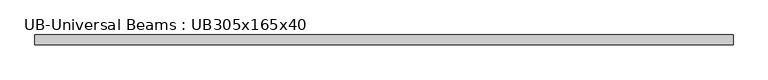
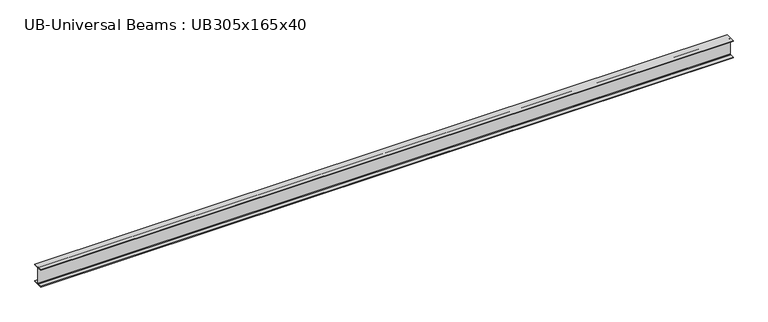
"""IFC4 building model written with IfcOpenShell, lengths in millimetres: member geometry, UB-Universal Beams : UB305x165x40."""

from ifc_helpers import new_model, si_unit, point, frame, frame_2d, origin, place, context, project, spatial, polyline, circle_curve, trimmed, segment, composite_curve, outline, extrude, source, transform, mapped, element, save


def ub_universal_beams_ub305x165x40_eee0c611(model_context):
    return source(origin(), model_context, "Body", "SweptSolid", [
        extrude(outline(composite_curve([segment(polyline([(82.5, -141.5), (82.5, -151.7), (-82.5, -151.7), (-82.5, -141.5), (-11.9, -141.5)]), True, "CONTINUOUS"), segment(trimmed(circle_curve(frame_2d((-11.9, -132.6)), 8.9), [point((-11.9, -141.5))], [point((-3.0, -132.6))], True, "CARTESIAN"), True, "CONTINUOUS"), segment(polyline([(-3.0, -132.6), (-3.0, 132.6)]), True, "CONTINUOUS"), segment(trimmed(circle_curve(frame_2d((-11.9, 132.6)), 8.9), [point((-3.0, 132.6))], [point((-11.9, 141.5))], True, "CARTESIAN"), True, "CONTINUOUS"), segment(polyline([(-11.9, 141.5), (-82.5, 141.5), (-82.5, 151.7), (82.5, 151.7), (82.5, 141.5), (11.9, 141.5)]), True, "CONTINUOUS"), segment(trimmed(circle_curve(frame_2d((11.9, 132.6)), 8.9), [point((11.9, 141.5))], [point((3.0, 132.6))], True, "CARTESIAN"), True, "CONTINUOUS"), segment(polyline([(3.0, 132.6), (3.0, -132.6)]), True, "CONTINUOUS"), segment(trimmed(circle_curve(frame_2d((11.9, -132.6)), 8.9), [point((3.0, -132.6))], [point((11.9, -141.5))], True, "CARTESIAN"), True, "CONTINUOUS"), segment(polyline([(11.9, -141.5), (82.5, -141.5)]), True, "CONTINUOUS")], self_intersect=False)), frame((-5621.7, 0.0, 0.0), z_axis=(1.0, 0.0, 0.0), x_axis=(0.0, 1.0, 0.0)), (0.0, 0.0, 1.0), 11577.5),
    ])


if __name__ == "__main__":
    model = new_model("IFC4")
    model_context = context("Model", 3, world=origin())
    ifc_project = project(units=[si_unit("LENGTHUNIT", "METRE", prefix="MILLI")], contexts=[model_context])
    site = spatial("IfcSite", under=ifc_project)
    building = spatial("IfcBuilding", under=site)
    placement = place(None, origin())
    ub_universal_beams_ub305x165x40_shape = ub_universal_beams_ub305x165x40_eee0c611(model_context)
    element("IfcMember", 1, ObjectType="UB-Universal Beams : UB305x165x40", at=placement, inside=building, context=model_context, shape_type="MappedRepresentation", body=[
        mapped(ub_universal_beams_ub305x165x40_shape, transform((0.0, 0.0, 0.0), x_axis=(1.0, 0.0, 0.0), y_axis=(0.0, 1.0, 0.0), z_axis=(0.0, 0.0, 1.0))),
    ])
    save(model, "model.ifc")

# Revit data of these elements
# Type "UB-Universal Beams : UB305x165x40"
#   Section Name Key = "UB305X165X40"
#   Width = 16.5 cm
#   Web Thickness = 0.6 cm
#   Web Fillet = 0.89 cm
#   Warping Constant = 164000.0 cm⁶
#   Torsional Moment of Inertia = 14.70 cm⁴
#   Section Area = 51.3 cm²
#   Plastic Modulus weak axis = 142.0 cm³
#   Plastic Modulus strong axis = 623.0 cm³
#   Nominal Weight = 40.2999 kgf/m
#   Moment of Inertia weak axis = 764.00 cm⁴
#   Moment of Inertia strong axis = 8503.00 cm⁴
#   Height = 30.34 cm
#   Flange Thickness = 1.02 cm
#   Elastic Modulus weak axis = 92.6 cm³
#   Elastic Modulus strong axis = 560.0 cm³
#   Centroid Vertical = 15.17 cm
#   Centroid Horizontal = 8.25 cm
#   Bolt Spacing = 9.0 cm
#   Length [instance default] = 1500 mm
#   Structural Material [instance default] = Metal - Steel 43-275
#   Type Comments = ""
#   Assembly Code = ""
# Element 1 (IfcMember, "UB-Universal Beams : UB305x165x40")
#   Materials on its faces: "Metal - Steel 43-275"
# Materials
#   "Metal - Steel 43-275": class "Metal", colour RGB 247 247 247, transparency 0, Cost = 0
